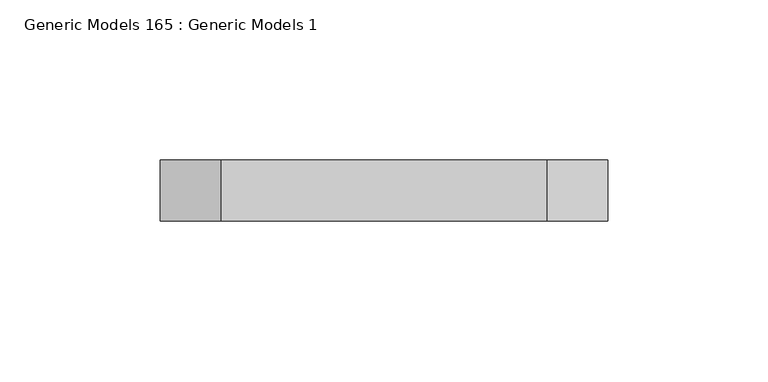
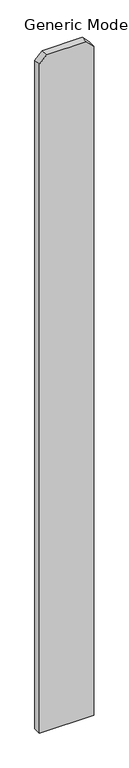
"""IFC4 building model written with IfcOpenShell, lengths in millimetres: proxy geometry, Generic Models 165 : Generic Models 1."""

import ifcopenshell
import ifcopenshell.guid

model = None  # the IFC model being written
_history = None  # IfcOwnerHistory: only IFC2X3 demands one
_inside = {}  # id of a spatial element -> (the spatial element, [elements in it])
_under = {}  # id of a project, library or spatial element -> (it, [spatial elements below it])
_declared = {}  # id of a project -> (the project, [libraries it declares])
_typed = {}  # id of a type object -> (the type object, [elements of that type])
_made_of = {}  # id of a material, layer set ... -> (it, [elements and type objects made of it])


def new_model(schema):
    """Start an empty IFC model of exactly this schema.

    Asked for "IFC4X3", IfcOpenShell would pick the latest addendum, in which some entities
    have other attributes; the version numbers below select the first issue.
    IFC2X3 requires an IfcOwnerHistory on every rooted entity: one is made here for all.
    """
    global model, _history
    if schema == "IFC4X3":
        model = ifcopenshell.file(schema_version=(4, 3, 0, 0))
    else:
        model = ifcopenshell.file(schema=schema)
    _inside.clear()
    _under.clear()
    _declared.clear()
    _typed.clear()
    _made_of.clear()
    _history = None
    if model.schema == "IFC2X3":
        org = make("IfcOrganization", Name="unknown")
        user = make(
            "IfcPersonAndOrganization",
            ThePerson=make("IfcPerson", FamilyName="unknown"),
            TheOrganization=org,
        )
        app = make(
            "IfcApplication",
            ApplicationDeveloper=org,
            Version="unknown",
            ApplicationFullName="unknown",
            ApplicationIdentifier="unknown",
        )
        _history = make(
            "IfcOwnerHistory",
            OwningUser=user,
            OwningApplication=app,
            ChangeAction="ADDED",
            CreationDate=0,
        )
    return model


def make(cls, **values):
    """One entity of the class cls with the attributes given. An attribute that is None is left unset."""
    return model.create_entity(
        cls, **{name: value for name, value in values.items() if value is not None}
    )


def rooted(cls, **values):
    """An entity with a GlobalId (a new one), such as an element, a storey or a relation."""
    return make(cls, GlobalId=ifcopenshell.guid.new(), OwnerHistory=_history, **values)


def si_unit(unit_type, name, prefix=None):
    """IfcSIUnit, for example si_unit("LENGTHUNIT", "METRE", prefix="MILLI")."""
    return make("IfcSIUnit", UnitType=unit_type, Prefix=prefix, Name=name)


def assignment(units):
    """IfcUnitAssignment: the units of a project."""
    return None if units is None else make("IfcUnitAssignment", Units=units)


def point(xyz):
    """IfcCartesianPoint."""
    return None if xyz is None else make("IfcCartesianPoint", Coordinates=xyz)


def direction(xyz):
    """IfcDirection."""
    return None if xyz is None else make("IfcDirection", DirectionRatios=xyz)


def frame(location, z_axis=None, x_axis=None):
    """IfcAxis2Placement3D, a coordinate frame: its origin and axes. An axis left out is left unset."""
    return make(
        "IfcAxis2Placement3D",
        Location=point(location),
        Axis=direction(z_axis),
        RefDirection=direction(x_axis),
    )


def origin():
    """The frame at (0, 0, 0) with its axes left unset."""
    return frame((0.0, 0.0, 0.0))


def place(relative_to, where):
    """IfcLocalPlacement: puts the frame where relative to a parent placement (None: the world)."""
    return make(
        "IfcLocalPlacement", PlacementRelTo=relative_to, RelativePlacement=where
    )


def context(
    kind, dimensions, precision=None, world=None, true_north=None, identifier=None
):
    """IfcGeometricRepresentationContext, for example the 3D "Model" context."""
    return make(
        "IfcGeometricRepresentationContext",
        ContextIdentifier=identifier,
        ContextType=kind,
        CoordinateSpaceDimension=dimensions,
        Precision=precision,
        WorldCoordinateSystem=world,
        TrueNorth=true_north,
    )


def project(units=None, contexts=None):
    """IfcProject with its units and contexts."""
    return rooted(
        "IfcProject",
        Name="project",
        RepresentationContexts=contexts,
        UnitsInContext=assignment(units),
    )


def spatial(cls, under=None, at=None, **own):
    """A site, building, storey or space (cls), placed at a placement, below another one or the project."""
    s = rooted(cls, ObjectPlacement=at, **own)
    if under is not None:
        _under.setdefault(under.id(), (under, []))[1].append(s)
    return s


def polyline(points):
    """IfcPolyline through the points."""
    return make("IfcPolyline", Points=[point(p) for p in points])


def outline(outer, holes=None, kind="AREA"):
    """IfcArbitraryClosedProfileDef: a profile drawn as a closed curve; with holes, ...WithVoids."""
    if holes is None:
        return make("IfcArbitraryClosedProfileDef", ProfileType=kind, OuterCurve=outer)
    return make(
        "IfcArbitraryProfileDefWithVoids",
        ProfileType=kind,
        OuterCurve=outer,
        InnerCurves=holes,
    )


def extrude(swept, where, along, depth):
    """IfcExtrudedAreaSolid: the profile swept, set in the frame where, extruded along a direction by depth."""
    return make(
        "IfcExtrudedAreaSolid",
        SweptArea=swept,
        Position=where,
        ExtrudedDirection=direction(along),
        Depth=depth,
    )


def shape(context_of_items, identifier, shape_type, items):
    """IfcShapeRepresentation: the items that make up one representation, for example the "Body"."""
    return make(
        "IfcShapeRepresentation",
        ContextOfItems=context_of_items,
        RepresentationIdentifier=identifier,
        RepresentationType=shape_type,
        Items=items,
    )


def source(mapping_origin, context_of_items, identifier, shape_type, items):
    """IfcRepresentationMap: a shape defined once, which mapped items show again and again."""
    return make(
        "IfcRepresentationMap",
        MappingOrigin=mapping_origin,
        MappedRepresentation=shape(context_of_items, identifier, shape_type, items),
    )


def transform(
    local_origin,
    x_axis=None,
    y_axis=None,
    z_axis=None,
    scale=None,
    scale2=None,
    scale3=None,
    uniform=True,
):
    """IfcCartesianTransformationOperator3D, or its non-uniform kind. x_axis, y_axis, z_axis: its Axis1, 2, 3."""
    if uniform:
        return make(
            "IfcCartesianTransformationOperator3D",
            Axis1=direction(x_axis),
            Axis2=direction(y_axis),
            LocalOrigin=point(local_origin),
            Scale=scale,
            Axis3=direction(z_axis),
        )
    return make(
        "IfcCartesianTransformationOperator3DnonUniform",
        Axis1=direction(x_axis),
        Axis2=direction(y_axis),
        LocalOrigin=point(local_origin),
        Scale=scale,
        Axis3=direction(z_axis),
        Scale2=scale2,
        Scale3=scale3,
    )


def mapped(mapping_source, mapping_target):
    """IfcMappedItem: shows the shape of a source again, moved by a transform."""
    return make(
        "IfcMappedItem", MappingSource=mapping_source, MappingTarget=mapping_target
    )


def made_of(thing, what):
    """Note that an element or type object is made of a material, layer set ...; save() writes the relation."""
    if what is not None:
        _made_of.setdefault(what.id(), (what, []))[1].append(thing)
    return thing


def element(
    cls,
    number,
    at=None,
    inside=None,
    cuts=None,
    type_object=None,
    material=None,
    context=None,
    identifier="Body",
    shape_type=None,
    held_by="IfcProductDefinitionShape",
    body=None,
    shapes=None,
    **own,
):
    """One element of the class cls, such as IfcWall. Its Tag is "e" and its number.

    at: its placement. inside: the storey or other place that contains it. cuts: it is an
    opening in that element (IfcRelVoidsElement). A single representation is given by context,
    identifier, shape_type and body (its items); several are given by shapes. held_by: the class
    of the entity that holds the representations. save() writes the other relations.
    """
    e = rooted(cls, Tag="e%d" % number, ObjectPlacement=at, **own)
    if body is not None:
        shapes = [shape(context, identifier, shape_type, body)]
    if shapes is not None:
        e.Representation = make(held_by, Representations=shapes)
    if inside is not None:
        _inside.setdefault(inside.id(), (inside, []))[1].append(e)
    if cuts is not None:
        rooted(
            "IfcRelVoidsElement", RelatingBuildingElement=cuts, RelatedOpeningElement=e
        )
    if type_object is not None:
        _typed.setdefault(type_object.id(), (type_object, []))[1].append(e)
    return made_of(e, material)


def aggregate(whole, parts):
    """IfcRelAggregates: a whole, such as a stair, and the parts it consists of."""
    return rooted("IfcRelAggregates", RelatingObject=whole, RelatedObjects=parts)


def save(model, path):
    """Write the relations noted so far, then the file.

    IfcRelAggregates (storeys below a building ...), IfcRelContainedInSpatialStructure (elements
    in a storey), IfcRelDefinesByType, IfcRelAssociatesMaterial and IfcRelDeclares: one each for
    every whole, place, type object, material and project.
    """
    for whole, parts in _under.values():
        aggregate(whole, parts)
    for where, things in _inside.values():
        rooted(
            "IfcRelContainedInSpatialStructure",
            RelatedElements=things,
            RelatingStructure=where,
        )
    for kind, things in _typed.values():
        rooted("IfcRelDefinesByType", RelatedObjects=things, RelatingType=kind)
    for what, things in _made_of.values():
        rooted("IfcRelAssociatesMaterial", RelatedObjects=things, RelatingMaterial=what)
    for by, libraries in _declared.values():
        rooted("IfcRelDeclares", RelatingContext=by, RelatedDefinitions=libraries)
    model.write(path)


def generic_models_165_generic_models_1_5258939b(model_context):
    return source(origin(), model_context, "Body", "SweptSolid", [
        extrude(outline(polyline([(76.2, -249658.1875), (1885.95, -249658.1875), (1905.0, -249677.2375), (1905.0, -249778.8375), (1885.95, -249797.8875), (76.2, -249797.8875), (76.2, -249658.1875)])), frame((0.0, 547.6875, 0.0), z_axis=(0.0, 1.0, 0.0), x_axis=(0.0, 0.0, 1.0)), (0.0, 0.0, 1.0), 19.05),
    ])


if __name__ == "__main__":
    model = new_model("IFC4")
    model_context = context("Model", 3, world=origin())
    ifc_project = project(units=[si_unit("LENGTHUNIT", "METRE", prefix="MILLI")], contexts=[model_context])
    site = spatial("IfcSite", under=ifc_project)
    building = spatial("IfcBuilding", under=site)
    placement = place(None, origin())
    generic_models_165_generic_models_1_shape = generic_models_165_generic_models_1_5258939b(model_context)
    element("IfcBuildingElementProxy", 1, Name="Generic Models 165 : Generic Models 1", ObjectType="Generic Models 165 : Generic Models 1", at=placement, inside=building, context=model_context, shape_type="MappedRepresentation", body=[
        mapped(generic_models_165_generic_models_1_shape, transform((0.0, 0.0, 0.0), x_axis=(1.0, 0.0, 0.0), y_axis=(0.0, 1.0, 0.0), z_axis=(0.0, 0.0, 1.0))),
    ])
    save(model, "model.ifc")

# Revit data of these elements
# Element 1 (IfcBuildingElementProxy, "Generic Models 165 : Generic Models 1")
#   Materials on its faces: "VERTICAL 1X6 CEDAR PLANKS W/ CLEAR WOOD SEALER"
# Materials
#   "VERTICAL 1X6 CEDAR PLANKS W/ CLEAR WOOD SEALER": class "Wood", colour RGB 234 198 147, transparency 0, Description = "Pinus Echinata", Cost = 0
